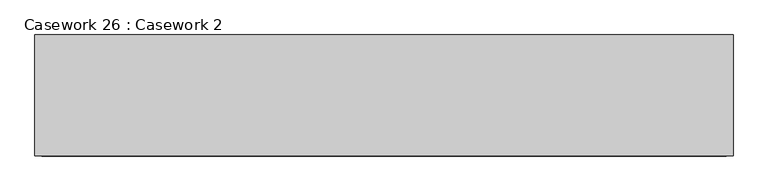
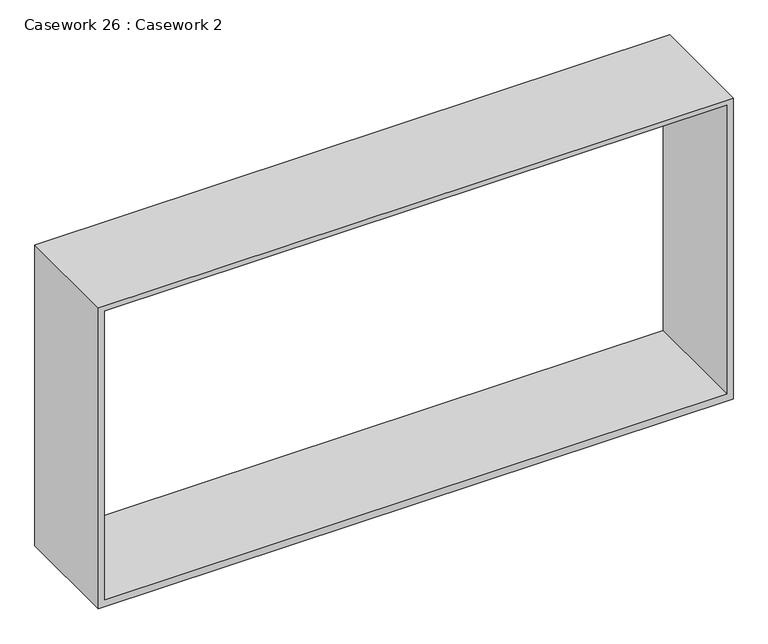
"""IFC4 building model written with IfcOpenShell, lengths in millimetres: furniture geometry, Casework 26 : Casework 2."""

from ifc_helpers import new_model, si_unit, frame, origin, place, context, project, spatial, polyline, outline, extrude, source, transform, mapped, element, save


def casework_26_casework_2_64ae3703(model_context):
    return source(origin(), model_context, "Body", "SweptSolid", [
        extrude(outline(polyline([(3048.0, -44729.8696714), (1745.7153081, -44729.8696714), (1745.7153081, -42133.813494), (3048.0, -42133.813494), (3048.0, -44729.8696714)]), holes=[polyline([(3024.850107, -44704.4696714), (3024.850107, -42159.1275026), (1776.6383668, -42159.1275026), (1776.6383668, -44704.4696714), (3024.850107, -44704.4696714)])]), frame((0.0, 285614.3720148, 0.0), z_axis=(0.0, 1.0, 0.0), x_axis=(0.0, 0.0, 1.0)), (0.0, 0.0, 1.0), 450.1962661),
    ])


if __name__ == "__main__":
    model = new_model("IFC4")
    model_context = context("Model", 3, world=origin())
    ifc_project = project(units=[si_unit("LENGTHUNIT", "METRE", prefix="MILLI")], contexts=[model_context])
    site = spatial("IfcSite", under=ifc_project)
    building = spatial("IfcBuilding", under=site)
    placement = place(None, origin())
    casework_26_casework_2_shape = casework_26_casework_2_64ae3703(model_context)
    element("IfcFurniture", 1, ObjectType="Casework 26 : Casework 2", at=placement, inside=building, context=model_context, shape_type="MappedRepresentation", body=[
        mapped(casework_26_casework_2_shape, transform((0.0, 0.0, 0.0), x_axis=(1.0, 0.0, 0.0), y_axis=(0.0, 1.0, 0.0), z_axis=(0.0, 0.0, 1.0))),
    ])
    save(model, "model.ifc")

# Revit data of these elements
# Element 1 (IfcFurniture, "Casework 26 : Casework 2")
#   Materials on its faces: "ALUMINUM PROFILE AT POLYCARBONATE PANEL"
# Materials
#   "ALUMINUM PROFILE AT POLYCARBONATE PANEL": class "Metal", colour RGB 244 244 244, transparency 0, Description = "Aluminum 6061", Cost = 0
